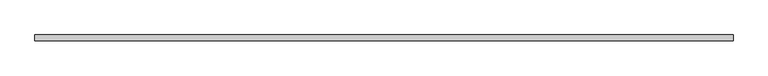
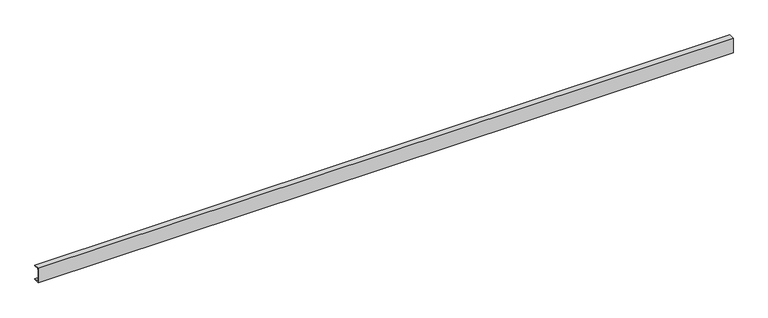
"""IFC4 building model written with IfcOpenShell, lengths in millimetres: beam geometry, С-образный профиль с параллельными полками (ГОСТ 8240-89) Балки : [ 20P."""

from ifc_helpers import new_model, si_unit, point, frame, frame_2d, origin, place, context, project, spatial, polyline, circle_curve, trimmed, segment, composite_curve, outline, extrude, source, transform, mapped, element, save


def beam_48740a10(model_context):
    return source(origin(), model_context, "Body", "SweptSolid", [
        extrude(outline(composite_curve([segment(polyline([(-23.0, 100.0), (53.0, 100.0), (53.0, 91.0), (-8.3, 91.0)]), True, "CONTINUOUS"), segment(trimmed(circle_curve(frame_2d((-8.3, 81.5)), 9.5), [point((-8.3, 91.0))], [point((-17.8, 81.5))], True, "CARTESIAN"), True, "CONTINUOUS"), segment(polyline([(-17.8, 81.5), (-17.8, -81.5)]), True, "CONTINUOUS"), segment(trimmed(circle_curve(frame_2d((-8.3, -81.5)), 9.5), [point((-17.8, -81.5))], [point((-8.3, -91.0))], True, "CARTESIAN"), True, "CONTINUOUS"), segment(polyline([(-8.3, -91.0), (53.0, -91.0), (53.0, -100.0), (-23.0, -100.0), (-23.0, 100.0)]), True, "CONTINUOUS")], self_intersect=False)), frame((-4585.0, 0.0, 0.0), z_axis=(1.0, 0.0, 0.0), x_axis=(0.0, 1.0, 0.0)), (0.0, 0.0, 1.0), 9170.0),
    ])


if __name__ == "__main__":
    model = new_model("IFC4")
    model_context = context("Model", 3, world=origin())
    ifc_project = project(units=[si_unit("LENGTHUNIT", "METRE", prefix="MILLI")], contexts=[model_context])
    site = spatial("IfcSite", under=ifc_project)
    building = spatial("IfcBuilding", under=site)
    placement = place(None, origin())
    beam_shape = beam_48740a10(model_context)
    element("IfcBeam", 1, ObjectType="С-образный профиль с параллельными полками (ГОСТ 8240-89) Балки : [ 20P", at=placement, inside=building, context=model_context, shape_type="MappedRepresentation", body=[
        mapped(beam_shape, transform((0.0, 0.0, 0.0), x_axis=(1.0, 0.0, 0.0), y_axis=(0.0, 1.0, 0.0), z_axis=(0.0, 0.0, 1.0))),
    ])
    save(model, "model.ifc")

# Revit data of these elements
# Type "С-образный профиль с параллельными полками (ГОСТ 8240-89) Балки : [ 20P"
#   tf = 9 mm
#   ra = 9.5 mm
#   W = 0.180442
#   Vz = 100 mm
#   Vy = 53 mm
#   Vpz = 100 mm
#   Vpy = 23 mm
#   Length [instance default] = 1500 mm
#   bf = 76 mm
#   d = 200 mm
#   tw = 5.2 mm
#   A = 0.00234 m²
#   Structural Material [instance default] = Металл - Сталь - 345 МПa
#   Assembly Code = ""
# Element 1 (IfcBeam, "С-образный профиль с параллельными полками (ГОСТ 8240-89) Балки : [ 20P")
#   Structural Material = C245
#   Materials on its faces: "C245"
# Materials
#   "Металл - Сталь - 345 МПa": class "Металл", colour RGB 247 247 247, transparency 0
#   "C245": class "Не назначено", colour RGB 0 0 0, transparency 0
